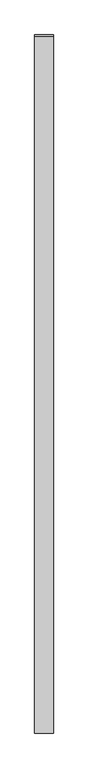
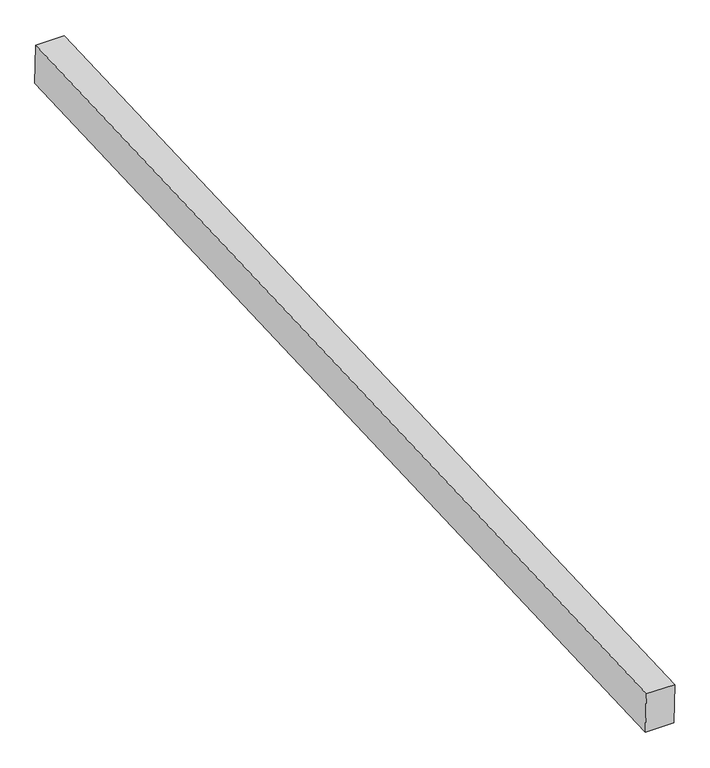
"""IFC4 building model written with IfcOpenShell, lengths in millimetres: proxy geometry, Generic Models 7:Generic Models 1:8:Generic Models 1:8 : Generic Models 7:Generic Models 1:337419:23 : Generic Models 7:Generic Models 1:8:Generic Models 1:8 : Generic Models 7:Generic Models 1:337419:315935."""

import ifcopenshell
import ifcopenshell.guid

model = None  # the IFC model being written
_history = None  # IfcOwnerHistory: only IFC2X3 demands one
_inside = {}  # id of a spatial element -> (the spatial element, [elements in it])
_under = {}  # id of a project, library or spatial element -> (it, [spatial elements below it])
_declared = {}  # id of a project -> (the project, [libraries it declares])
_typed = {}  # id of a type object -> (the type object, [elements of that type])
_made_of = {}  # id of a material, layer set ... -> (it, [elements and type objects made of it])


def new_model(schema):
    """Start an empty IFC model of exactly this schema.

    Asked for "IFC4X3", IfcOpenShell would pick the latest addendum, in which some entities
    have other attributes; the version numbers below select the first issue.
    IFC2X3 requires an IfcOwnerHistory on every rooted entity: one is made here for all.
    """
    global model, _history
    if schema == "IFC4X3":
        model = ifcopenshell.file(schema_version=(4, 3, 0, 0))
    else:
        model = ifcopenshell.file(schema=schema)
    _inside.clear()
    _under.clear()
    _declared.clear()
    _typed.clear()
    _made_of.clear()
    _history = None
    if model.schema == "IFC2X3":
        org = make("IfcOrganization", Name="unknown")
        user = make(
            "IfcPersonAndOrganization",
            ThePerson=make("IfcPerson", FamilyName="unknown"),
            TheOrganization=org,
        )
        app = make(
            "IfcApplication",
            ApplicationDeveloper=org,
            Version="unknown",
            ApplicationFullName="unknown",
            ApplicationIdentifier="unknown",
        )
        _history = make(
            "IfcOwnerHistory",
            OwningUser=user,
            OwningApplication=app,
            ChangeAction="ADDED",
            CreationDate=0,
        )
    return model


def make(cls, **values):
    """One entity of the class cls with the attributes given. An attribute that is None is left unset."""
    return model.create_entity(
        cls, **{name: value for name, value in values.items() if value is not None}
    )


def rooted(cls, **values):
    """An entity with a GlobalId (a new one), such as an element, a storey or a relation."""
    return make(cls, GlobalId=ifcopenshell.guid.new(), OwnerHistory=_history, **values)


def si_unit(unit_type, name, prefix=None):
    """IfcSIUnit, for example si_unit("LENGTHUNIT", "METRE", prefix="MILLI")."""
    return make("IfcSIUnit", UnitType=unit_type, Prefix=prefix, Name=name)


def assignment(units):
    """IfcUnitAssignment: the units of a project."""
    return None if units is None else make("IfcUnitAssignment", Units=units)


def point(xyz):
    """IfcCartesianPoint."""
    return None if xyz is None else make("IfcCartesianPoint", Coordinates=xyz)


def direction(xyz):
    """IfcDirection."""
    return None if xyz is None else make("IfcDirection", DirectionRatios=xyz)


def frame(location, z_axis=None, x_axis=None):
    """IfcAxis2Placement3D, a coordinate frame: its origin and axes. An axis left out is left unset."""
    return make(
        "IfcAxis2Placement3D",
        Location=point(location),
        Axis=direction(z_axis),
        RefDirection=direction(x_axis),
    )


def origin():
    """The frame at (0, 0, 0) with its axes left unset."""
    return frame((0.0, 0.0, 0.0))


def place(relative_to, where):
    """IfcLocalPlacement: puts the frame where relative to a parent placement (None: the world)."""
    return make(
        "IfcLocalPlacement", PlacementRelTo=relative_to, RelativePlacement=where
    )


def context(
    kind, dimensions, precision=None, world=None, true_north=None, identifier=None
):
    """IfcGeometricRepresentationContext, for example the 3D "Model" context."""
    return make(
        "IfcGeometricRepresentationContext",
        ContextIdentifier=identifier,
        ContextType=kind,
        CoordinateSpaceDimension=dimensions,
        Precision=precision,
        WorldCoordinateSystem=world,
        TrueNorth=true_north,
    )


def project(units=None, contexts=None):
    """IfcProject with its units and contexts."""
    return rooted(
        "IfcProject",
        Name="project",
        RepresentationContexts=contexts,
        UnitsInContext=assignment(units),
    )


def spatial(cls, under=None, at=None, **own):
    """A site, building, storey or space (cls), placed at a placement, below another one or the project."""
    s = rooted(cls, ObjectPlacement=at, **own)
    if under is not None:
        _under.setdefault(under.id(), (under, []))[1].append(s)
    return s


def polyline(points):
    """IfcPolyline through the points."""
    return make("IfcPolyline", Points=[point(p) for p in points])


def outline(outer, holes=None, kind="AREA"):
    """IfcArbitraryClosedProfileDef: a profile drawn as a closed curve; with holes, ...WithVoids."""
    if holes is None:
        return make("IfcArbitraryClosedProfileDef", ProfileType=kind, OuterCurve=outer)
    return make(
        "IfcArbitraryProfileDefWithVoids",
        ProfileType=kind,
        OuterCurve=outer,
        InnerCurves=holes,
    )


def extrude(swept, where, along, depth):
    """IfcExtrudedAreaSolid: the profile swept, set in the frame where, extruded along a direction by depth."""
    return make(
        "IfcExtrudedAreaSolid",
        SweptArea=swept,
        Position=where,
        ExtrudedDirection=direction(along),
        Depth=depth,
    )


def shape(context_of_items, identifier, shape_type, items):
    """IfcShapeRepresentation: the items that make up one representation, for example the "Body"."""
    return make(
        "IfcShapeRepresentation",
        ContextOfItems=context_of_items,
        RepresentationIdentifier=identifier,
        RepresentationType=shape_type,
        Items=items,
    )


def source(mapping_origin, context_of_items, identifier, shape_type, items):
    """IfcRepresentationMap: a shape defined once, which mapped items show again and again."""
    return make(
        "IfcRepresentationMap",
        MappingOrigin=mapping_origin,
        MappedRepresentation=shape(context_of_items, identifier, shape_type, items),
    )


def transform(
    local_origin,
    x_axis=None,
    y_axis=None,
    z_axis=None,
    scale=None,
    scale2=None,
    scale3=None,
    uniform=True,
):
    """IfcCartesianTransformationOperator3D, or its non-uniform kind. x_axis, y_axis, z_axis: its Axis1, 2, 3."""
    if uniform:
        return make(
            "IfcCartesianTransformationOperator3D",
            Axis1=direction(x_axis),
            Axis2=direction(y_axis),
            LocalOrigin=point(local_origin),
            Scale=scale,
            Axis3=direction(z_axis),
        )
    return make(
        "IfcCartesianTransformationOperator3DnonUniform",
        Axis1=direction(x_axis),
        Axis2=direction(y_axis),
        LocalOrigin=point(local_origin),
        Scale=scale,
        Axis3=direction(z_axis),
        Scale2=scale2,
        Scale3=scale3,
    )


def mapped(mapping_source, mapping_target):
    """IfcMappedItem: shows the shape of a source again, moved by a transform."""
    return make(
        "IfcMappedItem", MappingSource=mapping_source, MappingTarget=mapping_target
    )


def made_of(thing, what):
    """Note that an element or type object is made of a material, layer set ...; save() writes the relation."""
    if what is not None:
        _made_of.setdefault(what.id(), (what, []))[1].append(thing)
    return thing


def element(
    cls,
    number,
    at=None,
    inside=None,
    cuts=None,
    type_object=None,
    material=None,
    context=None,
    identifier="Body",
    shape_type=None,
    held_by="IfcProductDefinitionShape",
    body=None,
    shapes=None,
    **own,
):
    """One element of the class cls, such as IfcWall. Its Tag is "e" and its number.

    at: its placement. inside: the storey or other place that contains it. cuts: it is an
    opening in that element (IfcRelVoidsElement). A single representation is given by context,
    identifier, shape_type and body (its items); several are given by shapes. held_by: the class
    of the entity that holds the representations. save() writes the other relations.
    """
    e = rooted(cls, Tag="e%d" % number, ObjectPlacement=at, **own)
    if body is not None:
        shapes = [shape(context, identifier, shape_type, body)]
    if shapes is not None:
        e.Representation = make(held_by, Representations=shapes)
    if inside is not None:
        _inside.setdefault(inside.id(), (inside, []))[1].append(e)
    if cuts is not None:
        rooted(
            "IfcRelVoidsElement", RelatingBuildingElement=cuts, RelatedOpeningElement=e
        )
    if type_object is not None:
        _typed.setdefault(type_object.id(), (type_object, []))[1].append(e)
    return made_of(e, material)


def aggregate(whole, parts):
    """IfcRelAggregates: a whole, such as a stair, and the parts it consists of."""
    return rooted("IfcRelAggregates", RelatingObject=whole, RelatedObjects=parts)


def save(model, path):
    """Write the relations noted so far, then the file.

    IfcRelAggregates (storeys below a building ...), IfcRelContainedInSpatialStructure (elements
    in a storey), IfcRelDefinesByType, IfcRelAssociatesMaterial and IfcRelDeclares: one each for
    every whole, place, type object, material and project.
    """
    for whole, parts in _under.values():
        aggregate(whole, parts)
    for where, things in _inside.values():
        rooted(
            "IfcRelContainedInSpatialStructure",
            RelatedElements=things,
            RelatingStructure=where,
        )
    for kind, things in _typed.values():
        rooted("IfcRelDefinesByType", RelatedObjects=things, RelatingType=kind)
    for what, things in _made_of.values():
        rooted("IfcRelAssociatesMaterial", RelatedObjects=things, RelatingMaterial=what)
    for by, libraries in _declared.values():
        rooted("IfcRelDeclares", RelatingContext=by, RelatedDefinitions=libraries)
    model.write(path)


def generic_models_ee38cca4(model_context):
    return source(origin(), model_context, "Body", "SweptSolid", [
        extrude(outline(polyline([(0.0, -4876.8), (0.0, 0.0), (130.175, 0.0), (130.175, -4876.8), (0.0, -4876.8)])), frame((593799.9992243, -569702.1816815, 8511.7500907), z_axis=(0.0, -0.041630544707935736, 0.9991330730925289), x_axis=(-1.0, 0.0, 0.0)), (0.0, 0.0, 1.0), 190.5),
    ])


if __name__ == "__main__":
    model = new_model("IFC4")
    model_context = context("Model", 3, world=origin())
    ifc_project = project(units=[si_unit("LENGTHUNIT", "METRE", prefix="MILLI")], contexts=[model_context])
    site = spatial("IfcSite", under=ifc_project)
    building = spatial("IfcBuilding", under=site)
    placement = place(None, origin())
    generic_models_shape = generic_models_ee38cca4(model_context)
    element("IfcBuildingElementProxy", 1, Name="Generic Models 7:Generic Models 1:8:Generic Models 1:8 : Generic Models 7:Generic Models 1:337419:23 : Generic Models 7:Generic Models 1:8:Generic Models 1:8 : Generic Models 7:Generic Models 1:337419:315935", ObjectType="Generic Models 7:Generic Models 1:8:Generic Models 1:8 : Generic Models 7:Generic Models 1:337419:23 : Generic Models 7:Generic Models 1:8:Generic Models 1:8 : Generic Models 7:Generic Models 1:337419:315935", at=placement, inside=building, context=model_context, shape_type="MappedRepresentation", body=[
        mapped(generic_models_shape, transform((0.0, 0.0, 0.0), x_axis=(1.0, 0.0, 0.0), y_axis=(0.0, 1.0, 0.0), z_axis=(0.0, 0.0, 1.0))),
    ])
    save(model, "model.ifc")

# Revit data of these elements
# Type "Generic Models 7:Generic Models 1:8:Generic Models 1:8 : Generic Models 7:Generic Models 1:337419:23 : Generic Models 7:Generic Models 1:8:Generic Models 1:8 : Generic Models 7:Generic Models 1:337419:315935"
#   NameOverride = "Generic Models 7:Generic Models 1:8:Generic Models 1:8 : Generic Models 7:Generic Models 1:337419:315935"
#   ObjectTypeOverride = "Generic Models 1:8 : Generic Models 7:Generic Models 1:337419"
#   Reference = "Generic Models 1"
#   Tag = "315935"
# Element 1 (IfcBuildingElementProxy, "Generic Models 7:Generic Models 1:8:Generic Models 1:8 : Generic Models 7:Generic Models 1:337419:23 : Generic Models 7:Generic Models 1:8:Generic Models 1:8 : Generic Models 7:Generic Models 1:337419:315935")
#   Materials on its faces: "5 1/8\" X 7 1/2\" EXTERIOR GRADE GLULAM BEAMS (4'- 0 1/4\" O.C.)"
# Materials
#   "5 1/8\" X 7 1/2\" EXTERIOR GRADE GLULAM BEAMS (4'- 0 1/4\" O.C.)": class "Wood", colour RGB 183 134 68, transparency 0, Keynote = "M06181300.01", Description = "Pinus Echinata", Cost = 0
